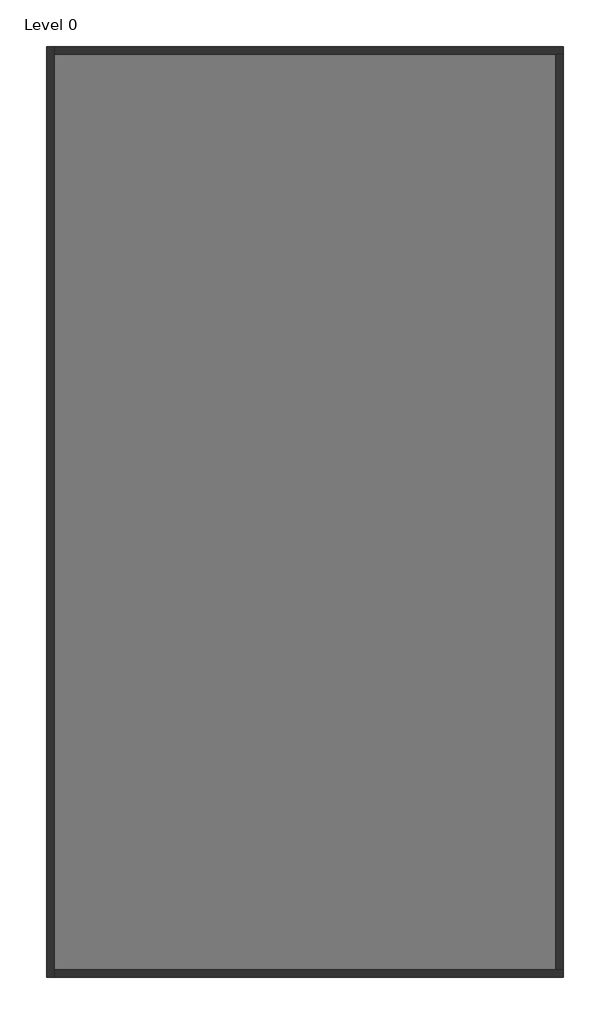
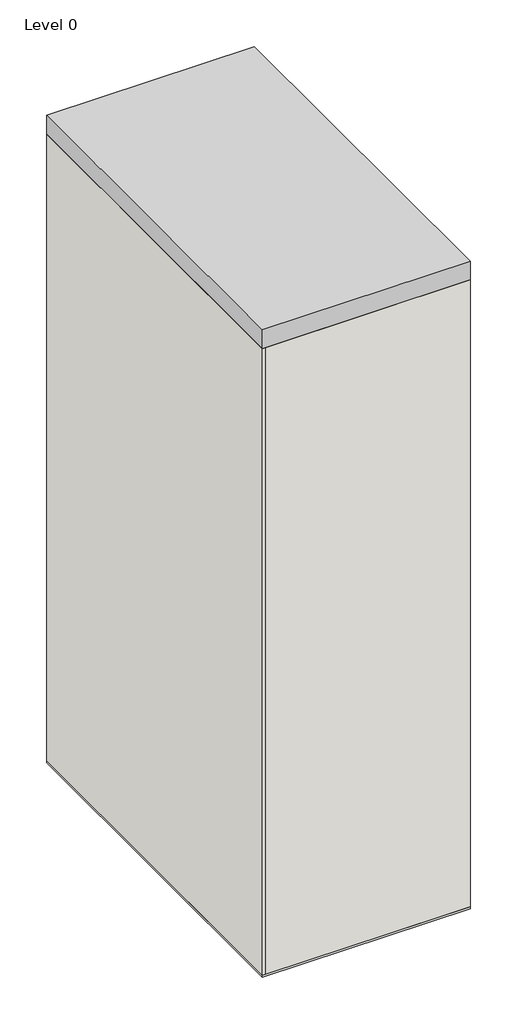
# One storey: 4 walls, 1 proxy, 1 slab.
"""IFC4 building model written with IfcOpenShell, lengths in millimetres."""

from ifc_helpers import new_model, si_unit, frame, origin, origin_with_axes, place, context, project, spatial, polyline, outline, extrude, faceted_brep, element, save

model = new_model("IFC4")

# Units and contexts
model_context = context("Model", 3, world=origin())
ifc_project = project(units=[si_unit("LENGTHUNIT", "METRE", prefix="MILLI")], contexts=[model_context])

# Site, building, storey
site = spatial("IfcSite", under=ifc_project)
building = spatial("IfcBuilding", under=site)
storey = spatial("IfcBuildingStorey", under=building, Name="Level 0", Elevation=100.0)

# Proxy
placement = place(None, origin())
element("IfcBuildingElementProxy", 1, Name="LowUrbanDensityBuilding : LowUrbanDensityBuilding", ObjectType="LowUrbanDensityBuilding : LowUrbanDensityBuilding", at=placement, inside=storey, context=model_context, shape_type="SweptSolid", body=[
    extrude(outline(polyline([(7325.2659446, 3676.2074539), (7325.2659446, -14323.7925461), (-2674.7340554, -14323.7925461), (-2674.7340554, 3676.2074539), (7325.2659446, 3676.2074539)])), origin_with_axes(), (0.0, 0.0, 1.0), 32949.8),
])

# Slab
element("IfcSlab", 2, ObjectType="Floor-Concrete_100Con", at=placement, inside=storey, context=model_context, shape_type="SweptSolid", body=[
    extrude(outline(polyline([(7325.2659446, 3676.2074539), (7325.2659446, -14323.7925461), (-2674.7340554, -14323.7925461), (-2674.7340554, 3676.2074539), (7325.2659446, 3676.2074539)])), origin_with_axes(), (0.0, 0.0, 1.0), 100.0),
])

# Walls
element("IfcWall", 3, ObjectType="Wall-Ext_25Rdr-100Blk-19P", at=placement, inside=storey, context=model_context, shape_type="Brep", body=[
    faceted_brep([(-2674.7340554, 3676.2074539, 100.0), (-2674.7340554, -14323.7925461, 100.0), (-2674.7340554, -14323.7925461, 32000.0), (-2674.7340554, 3676.2074539, 32000.0), (-2530.4340554, 3676.2074539, 100.0), (-2530.4340554, 3676.2074539, 32000.0), (-2530.4340554, 3531.9074539, 32000.0), (-2530.4340554, -14179.4925461, 32000.0), (-2530.4340554, -14323.7925461, 32000.0), (-2530.4340554, -14323.7925461, 100.0), (-2530.4340554, -14179.4925461, 100.0), (-2530.4340554, 3531.9074539, 100.0)], [[[0, 1, 2, 3]], [[4, 5, 6, 7, 8, 9, 10, 11]], [[1, 0, 4, 11, 10, 9]], [[3, 2, 8, 7, 6, 5]], [[2, 1, 9, 8]], [[0, 3, 5, 4]]]),
])
element("IfcWall", 4, ObjectType="Wall-Ext_25Rdr-100Blk-19P", at=placement, inside=storey, context=model_context, shape_type="Brep", body=[
    faceted_brep([(-2530.4340554, -14323.7925461, 100.0), (7325.2659446, -14323.7925461, 100.0), (7325.2659446, -14323.7925461, 32000.0), (-2530.4340554, -14323.7925461, 32000.0), (-2530.4340554, -14179.4925461, 100.0), (-2530.4340554, -14179.4925461, 32000.0), (7180.9659446, -14179.4925461, 32000.0), (7325.2659446, -14179.4925461, 32000.0), (7325.2659446, -14179.4925461, 100.0), (7180.9659446, -14179.4925461, 100.0)], [[[0, 1, 2, 3]], [[4, 5, 6, 7, 8, 9]], [[1, 0, 4, 9, 8]], [[3, 2, 7, 6, 5]], [[0, 3, 5, 4]], [[2, 1, 8, 7]]]),
])
element("IfcWall", 5, ObjectType="Wall-Ext_25Rdr-100Blk-19P", at=placement, inside=storey, context=model_context, shape_type="Brep", body=[
    faceted_brep([(7325.2659446, 3676.2074539, 100.0), (-2530.4340554, 3676.2074539, 100.0), (-2530.4340554, 3676.2074539, 32000.0), (7325.2659446, 3676.2074539, 32000.0), (7325.2659446, 3531.9074539, 100.0), (7325.2659446, 3531.9074539, 32000.0), (7180.9659446, 3531.9074539, 32000.0), (-2530.4340554, 3531.9074539, 32000.0), (-2530.4340554, 3531.9074539, 100.0), (7180.9659446, 3531.9074539, 100.0)], [[[0, 1, 2, 3]], [[4, 5, 6, 7, 8, 9]], [[1, 0, 4, 9, 8]], [[3, 2, 7, 6, 5]], [[2, 1, 8, 7]], [[0, 3, 5, 4]]]),
])
element("IfcWall", 6, ObjectType="Wall-Ext_25Rdr-100Blk-19P", at=placement, inside=storey, context=model_context, shape_type="SweptSolid", body=[
    extrude(outline(polyline([(7325.2659446, 3531.9074539), (7325.2659446, -14179.4925461), (7180.9659446, -14179.4925461), (7180.9659446, 3531.9074539), (7325.2659446, 3531.9074539)])), frame((0.0, 0.0, 100.0), z_axis=(0.0, 0.0, 1.0), x_axis=(1.0, 0.0, 0.0)), (0.0, 0.0, 1.0), 31900.0),
])

save(model, "model.ifc")

# Revit data of these elements
# Project information
#   Project Issue Date = "Issue Date"
#   Project Status = "Project Status"
#   Client Name = "Owner"
#   Project Address = "Enter address here"
#   Project Name = "Project Name"
#   Project Number = "Project Number"
# Type "Floor-Concrete_100Con"
#   Keynote = "E60/130"
#   Function = 0
#   Layers, outside or top first: 100 mm "Concrete" (function 1)
# Type "Wall-Ext_25Rdr-100Blk-19P"
#   Keynote = "F10"
#   Layers, outside or top first: 25.3 mm "Render, Beige, Smooth" (function 5); 100 mm "Concrete Masonry Units _Low Density" (function 1); 19 mm "Plaster" (function 5)
# Element 1 (IfcBuildingElementProxy, "LowUrbanDensityBuilding : LowUrbanDensityBuilding")
#   Phase Created = New Construction
#   Materials on its faces: "Default Form"
# Element 2 (IfcSlab, "Floor-Concrete_100Con")
#   Height Offset From Level = 0 mm
#   Phase Created = New Construction
#   Materials on its faces: "Concrete"
# Element 3 (IfcWall, "Wall-Ext_25Rdr-100Blk-19P")
#   Top Offset = 0 mm
#   Base Offset = 0 mm
#   wall height = 31900 mm
#   Phase Created = New Construction
#   Base Constraint = Level 0
#   Top Constraint = Level 8
#   Materials on its faces: "Render, Beige, Smooth", "Default Wall", "Plaster"
# Elements 4, 5, 6 (IfcWall, "Wall-Ext_25Rdr-100Blk-19P")
#   Top Offset = 0 mm
#   Base Offset = 0 mm
#   wall height = 31900 mm
#   Phase Created = New Construction
#   Base Constraint = Level 0
#   Top Constraint = Level 8
#   Materials on its faces: "Default Wall", "Render, Beige, Smooth", "Plaster"
# Materials
#   "Concrete": class "Concrete", colour RGB 120 120 120, transparency 0, Description = "Portland Cement Concrete", Cost = 0
#   "Render, Beige, Smooth": class "Generic", colour RGB 213 198 180, transparency 0, Description = "physical material", Cost = 0
#   "Concrete Masonry Units _Low Density": class "Masonry", colour RGB 181 181 181, transparency 0, Description = "Concrete masonry units", Cost = 0
#   "Plaster": class "Generic", colour RGB 249 249 249, transparency 0, Description = "Plaster", Cost = 0
#   "Default Form": class "Generic", colour RGB 185 189 196, transparency 0.5, Cost = 0
#   "Default Wall": class "Miscellaneous", colour RGB 128 128 128, transparency 0, Comments = "Rendering appearance not upgraded Rendering appearance not upgraded ", Cost = 0
